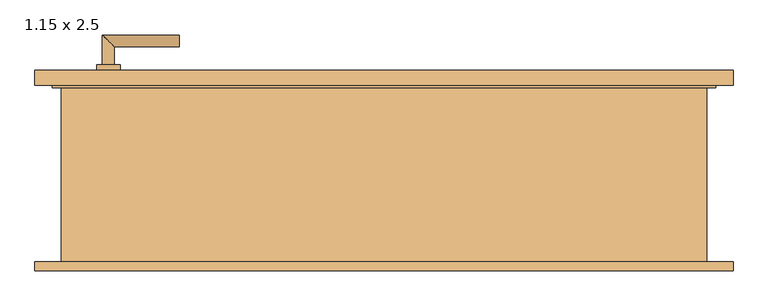
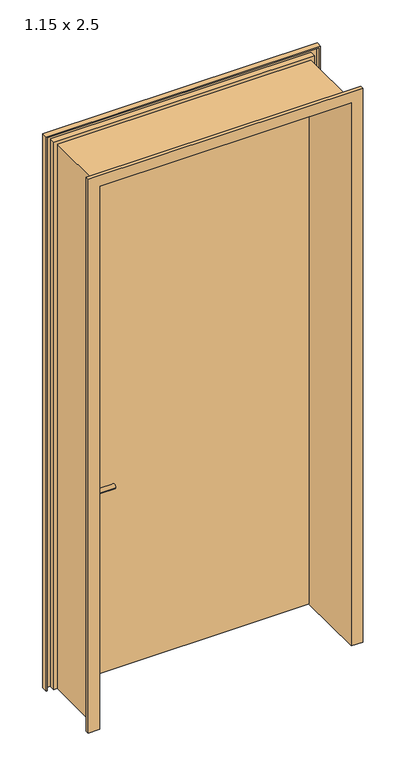
"""IFC4 building model written with IfcOpenShell, lengths in millimetres: door geometry, Drehflügel 1-flg - Stahlzarge : 1.15 x 2.5."""

import ifcopenshell
import ifcopenshell.guid

model = None  # the IFC model being written
_history = None  # IfcOwnerHistory: only IFC2X3 demands one
_inside = {}  # id of a spatial element -> (the spatial element, [elements in it])
_under = {}  # id of a project, library or spatial element -> (it, [spatial elements below it])
_declared = {}  # id of a project -> (the project, [libraries it declares])
_typed = {}  # id of a type object -> (the type object, [elements of that type])
_made_of = {}  # id of a material, layer set ... -> (it, [elements and type objects made of it])


def new_model(schema):
    """Start an empty IFC model of exactly this schema.

    Asked for "IFC4X3", IfcOpenShell would pick the latest addendum, in which some entities
    have other attributes; the version numbers below select the first issue.
    IFC2X3 requires an IfcOwnerHistory on every rooted entity: one is made here for all.
    """
    global model, _history
    if schema == "IFC4X3":
        model = ifcopenshell.file(schema_version=(4, 3, 0, 0))
    else:
        model = ifcopenshell.file(schema=schema)
    _inside.clear()
    _under.clear()
    _declared.clear()
    _typed.clear()
    _made_of.clear()
    _history = None
    if model.schema == "IFC2X3":
        org = make("IfcOrganization", Name="unknown")
        user = make(
            "IfcPersonAndOrganization",
            ThePerson=make("IfcPerson", FamilyName="unknown"),
            TheOrganization=org,
        )
        app = make(
            "IfcApplication",
            ApplicationDeveloper=org,
            Version="unknown",
            ApplicationFullName="unknown",
            ApplicationIdentifier="unknown",
        )
        _history = make(
            "IfcOwnerHistory",
            OwningUser=user,
            OwningApplication=app,
            ChangeAction="ADDED",
            CreationDate=0,
        )
    return model


def make(cls, **values):
    """One entity of the class cls with the attributes given. An attribute that is None is left unset."""
    return model.create_entity(
        cls, **{name: value for name, value in values.items() if value is not None}
    )


def rooted(cls, **values):
    """An entity with a GlobalId (a new one), such as an element, a storey or a relation."""
    return make(cls, GlobalId=ifcopenshell.guid.new(), OwnerHistory=_history, **values)


def si_unit(unit_type, name, prefix=None):
    """IfcSIUnit, for example si_unit("LENGTHUNIT", "METRE", prefix="MILLI")."""
    return make("IfcSIUnit", UnitType=unit_type, Prefix=prefix, Name=name)


def assignment(units):
    """IfcUnitAssignment: the units of a project."""
    return None if units is None else make("IfcUnitAssignment", Units=units)


def point(xyz):
    """IfcCartesianPoint."""
    return None if xyz is None else make("IfcCartesianPoint", Coordinates=xyz)


def direction(xyz):
    """IfcDirection."""
    return None if xyz is None else make("IfcDirection", DirectionRatios=xyz)


def frame(location, z_axis=None, x_axis=None):
    """IfcAxis2Placement3D, a coordinate frame: its origin and axes. An axis left out is left unset."""
    return make(
        "IfcAxis2Placement3D",
        Location=point(location),
        Axis=direction(z_axis),
        RefDirection=direction(x_axis),
    )


def frame_2d(location, x_axis=None):
    """IfcAxis2Placement2D, a coordinate frame in the plane: its origin and x axis."""
    return make(
        "IfcAxis2Placement2D", Location=point(location), RefDirection=direction(x_axis)
    )


def origin():
    """The frame at (0, 0, 0) with its axes left unset."""
    return frame((0.0, 0.0, 0.0))


def place(relative_to, where):
    """IfcLocalPlacement: puts the frame where relative to a parent placement (None: the world)."""
    return make(
        "IfcLocalPlacement", PlacementRelTo=relative_to, RelativePlacement=where
    )


def context(
    kind, dimensions, precision=None, world=None, true_north=None, identifier=None
):
    """IfcGeometricRepresentationContext, for example the 3D "Model" context."""
    return make(
        "IfcGeometricRepresentationContext",
        ContextIdentifier=identifier,
        ContextType=kind,
        CoordinateSpaceDimension=dimensions,
        Precision=precision,
        WorldCoordinateSystem=world,
        TrueNorth=true_north,
    )


def project(units=None, contexts=None):
    """IfcProject with its units and contexts."""
    return rooted(
        "IfcProject",
        Name="project",
        RepresentationContexts=contexts,
        UnitsInContext=assignment(units),
    )


def spatial(cls, under=None, at=None, **own):
    """A site, building, storey or space (cls), placed at a placement, below another one or the project."""
    s = rooted(cls, ObjectPlacement=at, **own)
    if under is not None:
        _under.setdefault(under.id(), (under, []))[1].append(s)
    return s


def polyline(points):
    """IfcPolyline through the points."""
    return make("IfcPolyline", Points=[point(p) for p in points])


def circle_curve(where, radius):
    """IfcCircle in the frame where."""
    return make("IfcCircle", Position=where, Radius=radius)


def ellipse_curve(where, semi_axis1, semi_axis2):
    """IfcEllipse in the frame where."""
    return make(
        "IfcEllipse", Position=where, SemiAxis1=semi_axis1, SemiAxis2=semi_axis2
    )


def trimmed(basis, trim1, trim2, sense, master):
    """IfcTrimmedCurve: the piece of a basis curve between two trims."""
    return make(
        "IfcTrimmedCurve",
        BasisCurve=basis,
        Trim1=trim1,
        Trim2=trim2,
        SenseAgreement=sense,
        MasterRepresentation=master,
    )


def segment(curve, same_sense, transition):
    """IfcCompositeCurveSegment."""
    return make(
        "IfcCompositeCurveSegment",
        Transition=transition,
        SameSense=same_sense,
        ParentCurve=curve,
    )


def composite_curve(segments, self_intersect=None):
    """IfcCompositeCurve: segments joined end to end."""
    return make("IfcCompositeCurve", Segments=segments, SelfIntersect=self_intersect)


def outline(outer, holes=None, kind="AREA"):
    """IfcArbitraryClosedProfileDef: a profile drawn as a closed curve; with holes, ...WithVoids."""
    if holes is None:
        return make("IfcArbitraryClosedProfileDef", ProfileType=kind, OuterCurve=outer)
    return make(
        "IfcArbitraryProfileDefWithVoids",
        ProfileType=kind,
        OuterCurve=outer,
        InnerCurves=holes,
    )


def extrude(swept, where, along, depth):
    """IfcExtrudedAreaSolid: the profile swept, set in the frame where, extruded along a direction by depth."""
    return make(
        "IfcExtrudedAreaSolid",
        SweptArea=swept,
        Position=where,
        ExtrudedDirection=direction(along),
        Depth=depth,
    )


def faces_of(points, faces, orient=None, outer=None):
    """IfcFace entities. A face is a list of loops; a loop is a list of indices into points, from 0.

    orient and outer hold one flag for each loop. By default every Orientation is true, the
    first loop of a face is its IfcFaceOuterBound and the others are IfcFaceBound.
    """
    made = []
    for i, loops in enumerate(faces):
        bounds = []
        for j, loop in enumerate(loops):
            is_outer = j == 0 if outer is None else outer[i][j]
            bounds.append(
                make(
                    "IfcFaceOuterBound" if is_outer else "IfcFaceBound",
                    Bound=make("IfcPolyLoop", Polygon=[points[k] for k in loop]),
                    Orientation=True if orient is None else orient[i][j],
                )
            )
        made.append(make("IfcFace", Bounds=bounds))
    return made


def faceted_brep(points, faces, orient=None, outer=None, voids=None):
    """IfcFacetedBrep: a solid bounded by flat faces; with voids (closed shells), ...WithVoids."""
    shared = [point(p) for p in points]
    hull = make("IfcClosedShell", CfsFaces=faces_of(shared, faces, orient, outer))
    if voids is None:
        return make("IfcFacetedBrep", Outer=hull)
    return make(
        "IfcFacetedBrepWithVoids",
        Outer=hull,
        Voids=[
            make(cls, CfsFaces=faces_of(shared, fs, o, b)) for cls, fs, o, b in voids
        ],
    )


def shape(context_of_items, identifier, shape_type, items):
    """IfcShapeRepresentation: the items that make up one representation, for example the "Body"."""
    return make(
        "IfcShapeRepresentation",
        ContextOfItems=context_of_items,
        RepresentationIdentifier=identifier,
        RepresentationType=shape_type,
        Items=items,
    )


def source(mapping_origin, context_of_items, identifier, shape_type, items):
    """IfcRepresentationMap: a shape defined once, which mapped items show again and again."""
    return make(
        "IfcRepresentationMap",
        MappingOrigin=mapping_origin,
        MappedRepresentation=shape(context_of_items, identifier, shape_type, items),
    )


def transform(
    local_origin,
    x_axis=None,
    y_axis=None,
    z_axis=None,
    scale=None,
    scale2=None,
    scale3=None,
    uniform=True,
):
    """IfcCartesianTransformationOperator3D, or its non-uniform kind. x_axis, y_axis, z_axis: its Axis1, 2, 3."""
    if uniform:
        return make(
            "IfcCartesianTransformationOperator3D",
            Axis1=direction(x_axis),
            Axis2=direction(y_axis),
            LocalOrigin=point(local_origin),
            Scale=scale,
            Axis3=direction(z_axis),
        )
    return make(
        "IfcCartesianTransformationOperator3DnonUniform",
        Axis1=direction(x_axis),
        Axis2=direction(y_axis),
        LocalOrigin=point(local_origin),
        Scale=scale,
        Axis3=direction(z_axis),
        Scale2=scale2,
        Scale3=scale3,
    )


def mapped(mapping_source, mapping_target):
    """IfcMappedItem: shows the shape of a source again, moved by a transform."""
    return make(
        "IfcMappedItem", MappingSource=mapping_source, MappingTarget=mapping_target
    )


def made_of(thing, what):
    """Note that an element or type object is made of a material, layer set ...; save() writes the relation."""
    if what is not None:
        _made_of.setdefault(what.id(), (what, []))[1].append(thing)
    return thing


def element(
    cls,
    number,
    at=None,
    inside=None,
    cuts=None,
    type_object=None,
    material=None,
    context=None,
    identifier="Body",
    shape_type=None,
    held_by="IfcProductDefinitionShape",
    body=None,
    shapes=None,
    **own,
):
    """One element of the class cls, such as IfcWall. Its Tag is "e" and its number.

    at: its placement. inside: the storey or other place that contains it. cuts: it is an
    opening in that element (IfcRelVoidsElement). A single representation is given by context,
    identifier, shape_type and body (its items); several are given by shapes. held_by: the class
    of the entity that holds the representations. save() writes the other relations.
    """
    e = rooted(cls, Tag="e%d" % number, ObjectPlacement=at, **own)
    if body is not None:
        shapes = [shape(context, identifier, shape_type, body)]
    if shapes is not None:
        e.Representation = make(held_by, Representations=shapes)
    if inside is not None:
        _inside.setdefault(inside.id(), (inside, []))[1].append(e)
    if cuts is not None:
        rooted(
            "IfcRelVoidsElement", RelatingBuildingElement=cuts, RelatedOpeningElement=e
        )
    if type_object is not None:
        _typed.setdefault(type_object.id(), (type_object, []))[1].append(e)
    return made_of(e, material)


def aggregate(whole, parts):
    """IfcRelAggregates: a whole, such as a stair, and the parts it consists of."""
    return rooted("IfcRelAggregates", RelatingObject=whole, RelatedObjects=parts)


def save(model, path):
    """Write the relations noted so far, then the file.

    IfcRelAggregates (storeys below a building ...), IfcRelContainedInSpatialStructure (elements
    in a storey), IfcRelDefinesByType, IfcRelAssociatesMaterial and IfcRelDeclares: one each for
    every whole, place, type object, material and project.
    """
    for whole, parts in _under.values():
        aggregate(whole, parts)
    for where, things in _inside.values():
        rooted(
            "IfcRelContainedInSpatialStructure",
            RelatedElements=things,
            RelatingStructure=where,
        )
    for kind, things in _typed.values():
        rooted("IfcRelDefinesByType", RelatedObjects=things, RelatingType=kind)
    for what, things in _made_of.values():
        rooted("IfcRelAssociatesMaterial", RelatedObjects=things, RelatingMaterial=what)
    for by, libraries in _declared.values():
        rooted("IfcRelDeclares", RelatingContext=by, RelatedDefinitions=libraries)
    model.write(path)


def plane_surface(at):
    """IfcPlane: the flat surface through the origin of the frame at, square to its z axis."""
    return make("IfcPlane", Position=at)


def cylinder_surface(at, radius):
    """IfcCylindricalSurface: all points at the distance radius from the z axis of the frame at."""
    return make("IfcCylindricalSurface", Position=at, Radius=radius)


def advanced_brep(points, edges, surfaces, faces):
    """IfcAdvancedBrep: a solid bounded by faces that lie on surfaces and meet in shared edges.

    An edge is (start, end): straight between two places in points (the first is 0);
    or (start, end, curve); or (start, end, curve, False) where it runs against its curve.
    A face is (place in surfaces, loops), or (place, loops, False) where it looks against
    its surface's normal. A loop lists edges by number (the first is 1), with a minus sign
    where the edge is run from its end to its start. The first loop is the outer one.
    """
    corners = [point(p) for p in points]
    vertices = [make("IfcVertexPoint", VertexGeometry=c) for c in corners]
    made = []
    for start, end, *more in edges:
        made.append(
            make(
                "IfcEdgeCurve",
                EdgeStart=vertices[start],
                EdgeEnd=vertices[end],
                EdgeGeometry=more[0] if more else make("IfcPolyline", Points=[corners[start], corners[end]]),
                SameSense=more[1] if len(more) > 1 else True,
            )
        )
    hull = []
    for where, loops, *sense in faces:
        bounds = []
        for j, loop in enumerate(loops):
            ring = [make("IfcOrientedEdge", EdgeElement=made[abs(k) - 1], Orientation=k > 0) for k in loop]
            bounds.append(
                make(
                    "IfcFaceOuterBound" if j == 0 else "IfcFaceBound",
                    Bound=make("IfcEdgeLoop", EdgeList=ring),
                    Orientation=True,
                )
            )
        hull.append(make("IfcAdvancedFace", Bounds=bounds, FaceSurface=surfaces[where], SameSense=sense[0] if sense else True))
    return make("IfcAdvancedBrep", Outer=make("IfcClosedShell", CfsFaces=hull))


def door_1_15_x_2_5_3229d866(model_context):
    return source(origin(), model_context, "Body", "SolidModel", [
        advanced_brep(
        [(-477.5, 139.4346141, 901.0), (-457.5, 139.4346141, 901.0), (-477.5, 69.4346141, 901.0), (-457.5, 89.4346141, 901.0), (-347.5, 69.4346141, 901.0), (-347.5, 89.4346141, 901.0)],
        [
            (0, 1, circle_curve(frame((-467.5, 139.4346141, 901.0), z_axis=(0.0, 1.0, 0.0), x_axis=(1.0, 0.0, 0.0)), 10.0)),
            (1, 0, circle_curve(frame((-467.5, 139.4346141, 901.0), z_axis=(0.0, 1.0, 0.0), x_axis=(1.0, 0.0, 0.0)), 10.0)),
            (0, 2),
            (2, 3, ellipse_curve(frame((-467.5, 79.4346141, 901.0), z_axis=(-0.7071067811865385, 0.7071067811865565, 0.0), x_axis=(0.7071067811865563, 0.7071067811865386, 0.0)), 14.1421356, 10.0)),
            (3, 1),
            (3, 2, ellipse_curve(frame((-467.5, 79.4346141, 901.0), z_axis=(-0.7071067811865385, 0.7071067811865565, 0.0), x_axis=(0.7071067811865563, 0.7071067811865386, 0.0)), 14.1421356, 10.0)),
            (4, 5, circle_curve(frame((-347.5, 79.4346141, 901.0), z_axis=(1.0, 0.0, 0.0), x_axis=(0.0, 1.0, 0.0)), 10.0)),
            (5, 4, circle_curve(frame((-347.5, 79.4346141, 901.0), z_axis=(1.0, 0.0, 0.0), x_axis=(0.0, 1.0, 0.0)), 10.0)),
            (2, 4),
            (5, 3),
        ],
        [
            plane_surface(frame((-467.5, 139.4346141, -386.7526403), z_axis=(0.0, 1.0, 0.0), x_axis=(0.0, 0.0, 1.0))),
            cylinder_surface(frame((-467.5, 139.4346141, 901.0), z_axis=(0.0, 1.0, 0.0), x_axis=(1.0, 0.0, 0.0)), 10.0),
            plane_surface(frame((-347.5, 79.4346141, -386.7526403), z_axis=(1.0, 0.0, 0.0), x_axis=(0.0, 0.0, 1.0))),
            cylinder_surface(frame((-467.5, 79.4346141, 901.0), z_axis=(-1.0, 0.0, 0.0), x_axis=(0.0, 1.0, 0.0)), 10.0),
        ],
        [
            (0, [[1, 2]]),
            (1, [[-1, 3, 4, 5]]),
            (1, [[-2, -5, 6, -3]]),
            (2, [[7, 8]]),
            (3, [[-4, 9, -8, 10]]),
            (3, [[-6, -10, -7, -9]]),
        ],
    ),
        advanced_brep(
        [(-457.5, 199.4346141, 901.0), (-477.5, 199.4346141, 901.0), (-457.5, 229.4346141, 901.0), (-477.5, 249.4346141, 901.0), (-347.5, 229.4346141, 901.0), (-347.5, 249.4346141, 901.0)],
        [
            (0, 1, circle_curve(frame((-467.5, 199.4346141, 901.0), z_axis=(0.0, -1.0, 0.0), x_axis=(-1.0, 0.0, 0.0)), 10.0)),
            (1, 0, circle_curve(frame((-467.5, 199.4346141, 901.0), z_axis=(0.0, -1.0, 0.0), x_axis=(-1.0, 0.0, 0.0)), 10.0)),
            (0, 2),
            (2, 3, ellipse_curve(frame((-467.5, 239.4346141, 901.0), z_axis=(-0.7071067811865475, -0.7071067811865475, 0.0), x_axis=(0.7071067811865474, -0.7071067811865476, 0.0)), 14.1421356, 10.0)),
            (3, 1),
            (3, 2, ellipse_curve(frame((-467.5, 239.4346141, 901.0), z_axis=(-0.7071067811865475, -0.7071067811865475, 0.0), x_axis=(0.7071067811865474, -0.7071067811865476, 0.0)), 14.1421356, 10.0)),
            (4, 5, circle_curve(frame((-347.5, 239.4346141, 901.0), z_axis=(1.0, 0.0, 0.0), x_axis=(0.0, 1.0, 0.0)), 10.0)),
            (5, 4, circle_curve(frame((-347.5, 239.4346141, 901.0), z_axis=(1.0, 0.0, 0.0), x_axis=(0.0, 1.0, 0.0)), 10.0)),
            (2, 4),
            (5, 3),
        ],
        [
            plane_surface(frame((-467.5, 199.4346141, -386.7526403), z_axis=(0.0, -1.0, 0.0), x_axis=(0.0, 0.0, 1.0))),
            cylinder_surface(frame((-467.5, 199.4346141, 901.0), z_axis=(0.0, -1.0, 0.0), x_axis=(-1.0, 0.0, 0.0)), 10.0),
            plane_surface(frame((-347.5, 239.4346141, -386.7526403), z_axis=(1.0, 0.0, 0.0), x_axis=(0.0, 0.0, 1.0))),
            cylinder_surface(frame((-467.5, 239.4346141, 901.0), z_axis=(-1.0, 0.0, 0.0), x_axis=(0.0, 1.0, 0.0)), 10.0),
        ],
        [
            (0, [[1, 2]]),
            (1, [[-1, 3, 4, 5]]),
            (1, [[-2, -5, 6, -3]]),
            (2, [[7, 8]]),
            (3, [[-4, 9, -8, 10]]),
            (3, [[-6, -10, -7, -9]]),
        ],
    ),
        extrude(outline(composite_curve([segment(trimmed(circle_curve(frame_2d((901.0, -467.5)), 20.0), [point((901.0, -487.5))], [point((901.0, -447.5))], False, "CARTESIAN"), True, "CONTINUOUS"), segment(trimmed(circle_curve(frame_2d((901.0, -467.5)), 20.0), [point((901.0, -447.5))], [point((901.0, -487.5))], False, "CARTESIAN"), True, "CONTINUOUS")], self_intersect=False)), frame((0.0, 129.4346141, 0.0), z_axis=(0.0, 1.0, 0.0), x_axis=(0.0, 0.0, 1.0)), (0.0, 0.0, 1.0), 10.0),
        extrude(outline(composite_curve([segment(trimmed(circle_curve(frame_2d((901.0, -467.5)), 20.0), [point((901.0, -487.5))], [point((901.0, -447.5))], False, "CARTESIAN"), True, "CONTINUOUS"), segment(trimmed(circle_curve(frame_2d((901.0, -467.5)), 20.0), [point((901.0, -447.5))], [point((901.0, -487.5))], False, "CARTESIAN"), True, "CONTINUOUS")], self_intersect=False)), frame((0.0, 189.4346141, 0.0), z_axis=(0.0, 1.0, 0.0), x_axis=(0.0, 0.0, 1.0)), (0.0, 0.0, 1.0), 10.0),
        extrude(outline(polyline([(557.5, 164.4346141), (-557.5, 164.4346141), (-557.5, 189.4346141), (557.5, 189.4346141), (557.5, 164.4346141)])), frame((0.0, 0.0, 1.0), z_axis=(0.0, 0.0, 1.0), x_axis=(1.0, 0.0, 0.0)), (0.0, 0.0, 1.0), 2490.0),
        faceted_brep([(591.9603207, -150.5653859, 1.0), (542.5, -150.5653859, 1.0), (542.5, 164.4346141, 1.0), (557.5, 164.4346141, 1.0), (557.5, 189.4346141, 1.0), (591.9603207, 189.4346141, 1.0), (591.9603207, 164.4346141, 1.0), (586.9603207, 164.4346141, 1.0), (586.9603207, 184.4346141, 1.0), (562.5, 184.4346141, 1.0), (562.5, 159.4346141, 1.0), (547.5, 159.4346141, 1.0), (547.5, -145.5653859, 1.0), (586.9603207, -145.5653859, 1.0), (586.9603207, -135.5653859, 1.0), (591.9603207, -135.5653859, 1.0), (591.9603207, -150.5653859, 2525.4603207), (-591.9603207, -150.5653859, 2525.4603207), (-591.9603207, -150.5653859, 1.0), (-542.5, -150.5653859, 1.0), (-542.5, -150.5653859, 2476.0), (542.5, -150.5653859, 2476.0), (542.5, 164.4346141, 2476.0), (-542.5, 164.4346141, 2476.0), (-542.5, 164.4346141, 1.0), (-557.5, 164.4346141, 1.0), (-557.5, 164.4346141, 2491.0), (557.5, 164.4346141, 2491.0), (557.5, 189.4346141, 2491.0), (-557.5, 189.4346141, 2491.0), (-557.5, 189.4346141, 1.0), (-591.9603207, 189.4346141, 1.0), (-591.9603207, 189.4346141, 2525.4603207), (591.9603207, 189.4346141, 2525.4603207), (591.9603207, 164.4346141, 2525.4603207), (-591.9603207, 164.4346141, 2525.4603207), (-591.9603207, 164.4346141, 1.0), (-586.9603207, 164.4346141, 1.0), (-586.9603207, 164.4346141, 2520.4603207), (586.9603207, 164.4346141, 2520.4603207), (586.9603207, 184.4346141, 2520.4603207), (-586.9603207, 184.4346141, 2520.4603207), (-586.9603207, 184.4346141, 1.0), (-562.5, 184.4346141, 1.0), (-562.5, 184.4346141, 2496.0), (562.5, 184.4346141, 2496.0), (562.5, 159.4346141, 2496.0), (-562.5, 159.4346141, 2496.0), (-562.5, 159.4346141, 1.0), (-547.5, 159.4346141, 1.0), (-547.5, 159.4346141, 2481.0), (547.5, 159.4346141, 2481.0), (547.5, -145.5653859, 2481.0), (-547.5, -145.5653859, 2481.0), (-547.5, -145.5653859, 1.0), (-586.9603207, -145.5653859, 1.0), (-586.9603207, -145.5653859, 2520.4603207), (586.9603207, -145.5653859, 2520.4603207), (586.9603207, -135.5653859, 2520.4603207), (-586.9603207, -135.5653859, 2520.4603207), (-586.9603207, -135.5653859, 1.0), (-591.9603207, -135.5653859, 1.0), (-591.9603207, -135.5653859, 2525.4603207), (591.9603207, -135.5653859, 2525.4603207)], [[[0, 1, 2, 3, 4, 5, 6, 7, 8, 9, 10, 11, 12, 13, 14, 15]], [[1, 0, 16, 17, 18, 19, 20, 21]], [[2, 1, 21, 22]], [[3, 2, 22, 23, 24, 25, 26, 27]], [[4, 3, 27, 28]], [[5, 4, 28, 29, 30, 31, 32, 33]], [[6, 5, 33, 34]], [[7, 6, 34, 35, 36, 37, 38, 39]], [[8, 7, 39, 40]], [[9, 8, 40, 41, 42, 43, 44, 45]], [[10, 9, 45, 46]], [[11, 10, 46, 47, 48, 49, 50, 51]], [[12, 11, 51, 52]], [[13, 12, 52, 53, 54, 55, 56, 57]], [[14, 13, 57, 58]], [[15, 14, 58, 59, 60, 61, 62, 63]], [[0, 15, 63, 16]], [[17, 62, 61, 18]], [[18, 61, 60, 55, 54, 49, 48, 43, 42, 37, 36, 31, 30, 25, 24, 19]], [[23, 20, 19, 24]], [[29, 26, 25, 30]], [[35, 32, 31, 36]], [[41, 38, 37, 42]], [[47, 44, 43, 48]], [[53, 50, 49, 54]], [[59, 56, 55, 60]], [[22, 21, 20, 23]], [[28, 27, 26, 29]], [[34, 33, 32, 35]], [[40, 39, 38, 41]], [[46, 45, 44, 47]], [[52, 51, 50, 53]], [[58, 57, 56, 59]], [[16, 63, 62, 17]]]),
    ])


if __name__ == "__main__":
    model = new_model("IFC4")
    model_context = context("Model", 3, world=origin())
    ifc_project = project(units=[si_unit("LENGTHUNIT", "METRE", prefix="MILLI")], contexts=[model_context])
    site = spatial("IfcSite", under=ifc_project)
    building = spatial("IfcBuilding", under=site)
    placement = place(None, origin())
    door_1_15_x_2_5_shape = door_1_15_x_2_5_3229d866(model_context)
    element("IfcDoor", 1, ObjectType="Drehflügel 1-flg - Stahlzarge : 1.15 x 2.5", at=placement, inside=building, context=model_context, shape_type="MappedRepresentation", body=[
        mapped(door_1_15_x_2_5_shape, transform((0.0, 0.0, 0.0), x_axis=(1.0, 0.0, 0.0), y_axis=(0.0, 1.0, 0.0), z_axis=(0.0, 0.0, 1.0))),
    ])
    save(model, "model.ifc")

# Revit data of these elements
# Type "Drehflügel 1-flg - Stahlzarge : 1.15 x 2.5"
#   Type Mark = "21"
#   Operation = "SingleSwingRight"
#   Keynote = "16.03"
#   Analytic Construction = "Metall"
#   Thermal Resistance (R) = 0.270117 (m²·K)/W
#   Heat Transfer Coefficient (U) = 3.7021 W/(m²·K)
#   Rough Width = 1.135 m
#   Rough Height [instance default] = 2.600 m
#   Höhe Türgriff [instance default] = 0.900 m
#   Height = 2.500 m
#   Fußbodenaufbau [instance default] = 0.100 m
#   Width = 1.135 m
#   Sichtbarkeit Sturzlinien [instance default] = yes
#   Türgriff auswählen [instance default] = element 221079
#   Türgriff [instance default] = none
#   Türflügel [instance default] = none
#   Rahmen/Pfosten [instance default] = Metall - Lackiert - Grau
#   Visual Light Transmittance = 0
#   Solar Heat Gain Coefficient = 0
#   Function = (empty or 0)
#   Wall Closure = (empty or 0)
# Element 1 (IfcDoor, "Drehflügel 1-flg - Stahlzarge : 1.15 x 2.5")
#   Rough Height = 2.501 m
#   Fußbodenaufbau = 0.001 m
#   Materials on its faces: "Metall - Lackiert - Grau", "Metall - Chrom", "Holz - Birke"
# Materials
#   "Metall - Lackiert - Grau": class "Farbe 1", colour RGB 98 98 98, transparency 0, Cost = 0
#   "Metall - Chrom": class "Metall", colour RGB 247 247 247, transparency 0, Cost = 0
#   "Holz - Birke": class "Holz", colour RGB 213 164 103, transparency 0, Cost = 0
